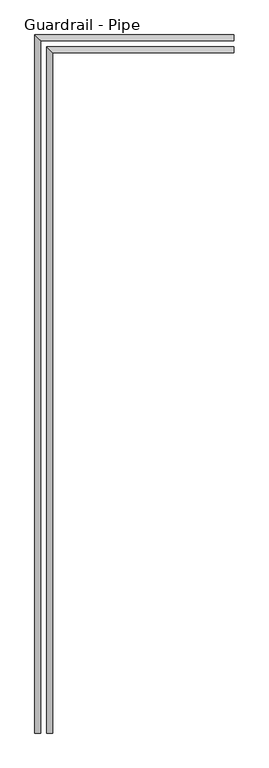
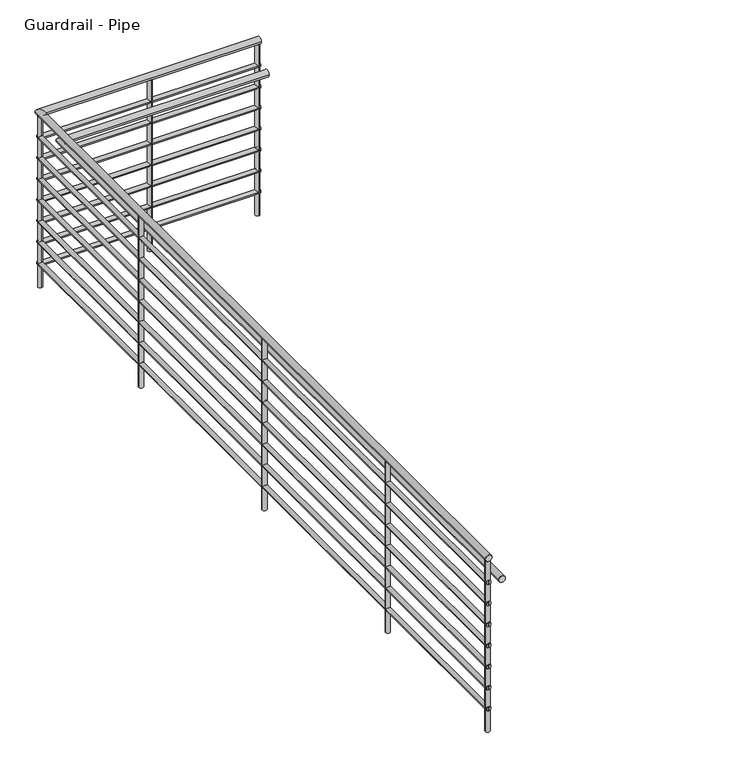
"""IFC4 building model written with IfcOpenShell, lengths in millimetres: railing geometry, Guardrail - Pipe."""

from ifc_helpers import new_model, si_unit, point, frame, frame_2d, origin, origin_with_axes, place, context, project, spatial, circle_curve, ellipse_curve, trimmed, segment, composite_curve, outline, extrude, source, transform, mapped, element, save
from ifc_brep_helpers import plane_surface, cylinder_surface, advanced_brep


def guardrail_pipe_2ce98fbd(model_context):
    return source(origin(), model_context, "Body", "SolidModel", [
        advanced_brep(
        [(-2073.0939612, 2865.859643, 1047.75), (-2073.0939612, 2903.959643, 1047.75), (-3304.9939612, 2865.859643, 1047.75), (-3343.0939612, 2903.959643, 1047.75), (-3304.9939612, -1546.6414366, 1047.75), (-3343.0939612, -1546.6414366, 1047.75)],
        [
            (0, 1, circle_curve(frame((-2073.0939612, 2884.909643, 1047.75), z_axis=(1.0, 0.0, 0.0), x_axis=(0.0, 1.0, 0.0)), 19.05)),
            (1, 0, circle_curve(frame((-2073.0939612, 2884.909643, 1047.75), z_axis=(1.0, 0.0, 0.0), x_axis=(0.0, 1.0, 0.0)), 19.05)),
            (0, 2),
            (2, 3, ellipse_curve(frame((-3324.0439612, 2884.909643, 1047.75), z_axis=(0.7071067811865492, 0.7071067811865458, 0.0), x_axis=(0.7071067811865458, -0.7071067811865492, 0.0)), 26.9407684, 19.05)),
            (3, 1),
            (3, 2, ellipse_curve(frame((-3324.0439612, 2884.909643, 1047.75), z_axis=(0.7071067811865492, 0.7071067811865458, 0.0), x_axis=(0.7071067811865458, -0.7071067811865492, 0.0)), 26.9407684, 19.05)),
            (4, 5, circle_curve(frame((-3324.0439612, -1546.6414366, 1047.75), z_axis=(0.0, -1.0, 0.0), x_axis=(-1.0, 0.0, 0.0)), 19.05)),
            (5, 4, circle_curve(frame((-3324.0439612, -1546.6414366, 1047.75), z_axis=(0.0, -1.0, 0.0), x_axis=(-1.0, 0.0, 0.0)), 19.05)),
            (2, 4),
            (5, 3),
        ],
        [
            plane_surface(frame((-2073.0939612, 2884.909643, 1066.8), z_axis=(1.0, 0.0, 0.0), x_axis=(0.0, -1.0, 0.0))),
            cylinder_surface(frame((-2073.0939612, 2884.909643, 1047.75), z_axis=(1.0, 0.0, 0.0), x_axis=(0.0, 1.0, 0.0)), 19.05),
            plane_surface(frame((-3324.0439612, -1546.6414366, 1066.8), z_axis=(0.0, -1.0, 0.0), x_axis=(0.0, 0.0, -1.0))),
            cylinder_surface(frame((-3324.0439612, 2884.909643, 1047.75), z_axis=(0.0, 1.0, 0.0), x_axis=(-1.0, 0.0, 0.0)), 19.05),
        ],
        [
            (0, [[1, 2]]),
            (1, [[-1, 3, 4, 5]]),
            (1, [[-2, -5, 6, -3]]),
            (2, [[7, 8]]),
            (3, [[-4, 9, -8, 10]]),
            (3, [[-6, -10, -7, -9]]),
        ],
    ),
        advanced_brep(
        [(-2073.0939612, 2872.209643, 901.7), (-2073.0939612, 2897.609643, 901.7), (-3311.3439612, 2872.209643, 901.7), (-3336.7439612, 2897.609643, 901.7), (-3311.3439612, -1546.6414366, 901.7), (-3336.7439612, -1546.6414366, 901.7)],
        [
            (0, 1, circle_curve(frame((-2073.0939612, 2884.909643, 901.7), z_axis=(1.0, 0.0, 0.0), x_axis=(0.0, 1.0, 0.0)), 12.7)),
            (1, 0, circle_curve(frame((-2073.0939612, 2884.909643, 901.7), z_axis=(1.0, 0.0, 0.0), x_axis=(0.0, 1.0, 0.0)), 12.7)),
            (0, 2),
            (2, 3, ellipse_curve(frame((-3324.0439612, 2884.909643, 901.7), z_axis=(0.7071067811865492, 0.7071067811865458, 0.0), x_axis=(0.7071067811865458, -0.7071067811865492, 0.0)), 17.9605122, 12.7)),
            (3, 1),
            (3, 2, ellipse_curve(frame((-3324.0439612, 2884.909643, 901.7), z_axis=(0.7071067811865492, 0.7071067811865458, 0.0), x_axis=(0.7071067811865458, -0.7071067811865492, 0.0)), 17.9605122, 12.7)),
            (4, 5, circle_curve(frame((-3324.0439612, -1546.6414366, 901.7), z_axis=(0.0, -1.0, 0.0), x_axis=(-1.0, 0.0, 0.0)), 12.7)),
            (5, 4, circle_curve(frame((-3324.0439612, -1546.6414366, 901.7), z_axis=(0.0, -1.0, 0.0), x_axis=(-1.0, 0.0, 0.0)), 12.7)),
            (2, 4),
            (5, 3),
        ],
        [
            plane_surface(frame((-2073.0939612, 2884.909643, 914.4), z_axis=(1.0, 0.0, 0.0), x_axis=(0.0, -1.0, 0.0))),
            cylinder_surface(frame((-2073.0939612, 2884.909643, 901.7), z_axis=(1.0, 0.0, 0.0), x_axis=(0.0, 1.0, 0.0)), 12.7),
            plane_surface(frame((-3324.0439612, -1546.6414366, 914.4), z_axis=(0.0, -1.0, 0.0), x_axis=(0.0, 0.0, -1.0))),
            cylinder_surface(frame((-3324.0439612, 2884.909643, 901.7), z_axis=(0.0, 1.0, 0.0), x_axis=(-1.0, 0.0, 0.0)), 12.7),
        ],
        [
            (0, [[1, 2]]),
            (1, [[-1, 3, 4, 5]]),
            (1, [[-2, -5, 6, -3]]),
            (2, [[7, 8]]),
            (3, [[-4, 9, -8, 10]]),
            (3, [[-6, -10, -7, -9]]),
        ],
    ),
        advanced_brep(
        [(-2073.0939612, 2789.659643, 895.35), (-2073.0939612, 2827.759643, 895.35), (-3228.7939612, 2789.659643, 895.35), (-3266.8939612, 2827.759643, 895.35), (-3228.7939612, -1546.6414366, 895.35), (-3266.8939612, -1546.6414366, 895.35)],
        [
            (0, 1, circle_curve(frame((-2073.0939612, 2808.709643, 895.35), z_axis=(1.0, 0.0, 0.0), x_axis=(0.0, 1.0, 0.0)), 19.05)),
            (1, 0, circle_curve(frame((-2073.0939612, 2808.709643, 895.35), z_axis=(1.0, 0.0, 0.0), x_axis=(0.0, 1.0, 0.0)), 19.05)),
            (0, 2),
            (2, 3, ellipse_curve(frame((-3247.8439612, 2808.709643, 895.35), z_axis=(0.7071067811865492, 0.7071067811865458, 0.0), x_axis=(0.7071067811865458, -0.7071067811865492, 0.0)), 26.9407684, 19.05)),
            (3, 1),
            (3, 2, ellipse_curve(frame((-3247.8439612, 2808.709643, 895.35), z_axis=(0.7071067811865492, 0.7071067811865458, 0.0), x_axis=(0.7071067811865458, -0.7071067811865492, 0.0)), 26.9407684, 19.05)),
            (4, 5, circle_curve(frame((-3247.8439612, -1546.6414366, 895.35), z_axis=(0.0, -1.0, 0.0), x_axis=(-1.0, 0.0, 0.0)), 19.05)),
            (5, 4, circle_curve(frame((-3247.8439612, -1546.6414366, 895.35), z_axis=(0.0, -1.0, 0.0), x_axis=(-1.0, 0.0, 0.0)), 19.05)),
            (2, 4),
            (5, 3),
        ],
        [
            plane_surface(frame((-2073.0939612, 2808.709643, 914.4), z_axis=(1.0, 0.0, 0.0), x_axis=(0.0, -1.0, 0.0))),
            cylinder_surface(frame((-2073.0939612, 2808.709643, 895.35), z_axis=(1.0, 0.0, 0.0), x_axis=(0.0, 1.0, 0.0)), 19.05),
            plane_surface(frame((-3247.8439612, -1546.6414366, 914.4), z_axis=(0.0, -1.0, 0.0), x_axis=(0.0, 0.0, -1.0))),
            cylinder_surface(frame((-3247.8439612, 2808.709643, 895.35), z_axis=(0.0, 1.0, 0.0), x_axis=(-1.0, 0.0, 0.0)), 19.05),
        ],
        [
            (0, [[1, 2]]),
            (1, [[-1, 3, 4, 5]]),
            (1, [[-2, -5, 6, -3]]),
            (2, [[7, 8]]),
            (3, [[-4, 9, -8, 10]]),
            (3, [[-6, -10, -7, -9]]),
        ],
    ),
        advanced_brep(
        [(-2073.0939612, 2872.209643, 774.7), (-2073.0939612, 2897.609643, 774.7), (-3311.3439612, 2872.209643, 774.7), (-3336.7439612, 2897.609643, 774.7), (-3311.3439612, -1546.6414366, 774.7), (-3336.7439612, -1546.6414366, 774.7)],
        [
            (0, 1, circle_curve(frame((-2073.0939612, 2884.909643, 774.7), z_axis=(1.0, 0.0, 0.0), x_axis=(0.0, 1.0, 0.0)), 12.7)),
            (1, 0, circle_curve(frame((-2073.0939612, 2884.909643, 774.7), z_axis=(1.0, 0.0, 0.0), x_axis=(0.0, 1.0, 0.0)), 12.7)),
            (0, 2),
            (2, 3, ellipse_curve(frame((-3324.0439612, 2884.909643, 774.7), z_axis=(0.7071067811865492, 0.7071067811865458, 0.0), x_axis=(0.7071067811865458, -0.7071067811865492, 0.0)), 17.9605122, 12.7)),
            (3, 1),
            (3, 2, ellipse_curve(frame((-3324.0439612, 2884.909643, 774.7), z_axis=(0.7071067811865492, 0.7071067811865458, 0.0), x_axis=(0.7071067811865458, -0.7071067811865492, 0.0)), 17.9605122, 12.7)),
            (4, 5, circle_curve(frame((-3324.0439612, -1546.6414366, 774.7), z_axis=(0.0, -1.0, 0.0), x_axis=(-1.0, 0.0, 0.0)), 12.7)),
            (5, 4, circle_curve(frame((-3324.0439612, -1546.6414366, 774.7), z_axis=(0.0, -1.0, 0.0), x_axis=(-1.0, 0.0, 0.0)), 12.7)),
            (2, 4),
            (5, 3),
        ],
        [
            plane_surface(frame((-2073.0939612, 2884.909643, 787.4), z_axis=(1.0, 0.0, 0.0), x_axis=(0.0, -1.0, 0.0))),
            cylinder_surface(frame((-2073.0939612, 2884.909643, 774.7), z_axis=(1.0, 0.0, 0.0), x_axis=(0.0, 1.0, 0.0)), 12.7),
            plane_surface(frame((-3324.0439612, -1546.6414366, 787.4), z_axis=(0.0, -1.0, 0.0), x_axis=(0.0, 0.0, -1.0))),
            cylinder_surface(frame((-3324.0439612, 2884.909643, 774.7), z_axis=(0.0, 1.0, 0.0), x_axis=(-1.0, 0.0, 0.0)), 12.7),
        ],
        [
            (0, [[1, 2]]),
            (1, [[-1, 3, 4, 5]]),
            (1, [[-2, -5, 6, -3]]),
            (2, [[7, 8]]),
            (3, [[-4, 9, -8, 10]]),
            (3, [[-6, -10, -7, -9]]),
        ],
    ),
        advanced_brep(
        [(-2073.0939612, 2872.209643, 647.7), (-2073.0939612, 2897.609643, 647.7), (-3311.3439612, 2872.209643, 647.7), (-3336.7439612, 2897.609643, 647.7), (-3311.3439612, -1546.6414366, 647.7), (-3336.7439612, -1546.6414366, 647.7)],
        [
            (0, 1, circle_curve(frame((-2073.0939612, 2884.909643, 647.7), z_axis=(1.0, 0.0, 0.0), x_axis=(0.0, 1.0, 0.0)), 12.7)),
            (1, 0, circle_curve(frame((-2073.0939612, 2884.909643, 647.7), z_axis=(1.0, 0.0, 0.0), x_axis=(0.0, 1.0, 0.0)), 12.7)),
            (0, 2),
            (2, 3, ellipse_curve(frame((-3324.0439612, 2884.909643, 647.7), z_axis=(0.7071067811865492, 0.7071067811865458, 0.0), x_axis=(0.7071067811865458, -0.7071067811865492, 0.0)), 17.9605122, 12.7)),
            (3, 1),
            (3, 2, ellipse_curve(frame((-3324.0439612, 2884.909643, 647.7), z_axis=(0.7071067811865492, 0.7071067811865458, 0.0), x_axis=(0.7071067811865458, -0.7071067811865492, 0.0)), 17.9605122, 12.7)),
            (4, 5, circle_curve(frame((-3324.0439612, -1546.6414366, 647.7), z_axis=(0.0, -1.0, 0.0), x_axis=(-1.0, 0.0, 0.0)), 12.7)),
            (5, 4, circle_curve(frame((-3324.0439612, -1546.6414366, 647.7), z_axis=(0.0, -1.0, 0.0), x_axis=(-1.0, 0.0, 0.0)), 12.7)),
            (2, 4),
            (5, 3),
        ],
        [
            plane_surface(frame((-2073.0939612, 2884.909643, 660.4), z_axis=(1.0, 0.0, 0.0), x_axis=(0.0, -1.0, 0.0))),
            cylinder_surface(frame((-2073.0939612, 2884.909643, 647.7), z_axis=(1.0, 0.0, 0.0), x_axis=(0.0, 1.0, 0.0)), 12.7),
            plane_surface(frame((-3324.0439612, -1546.6414366, 660.4), z_axis=(0.0, -1.0, 0.0), x_axis=(0.0, 0.0, -1.0))),
            cylinder_surface(frame((-3324.0439612, 2884.909643, 647.7), z_axis=(0.0, 1.0, 0.0), x_axis=(-1.0, 0.0, 0.0)), 12.7),
        ],
        [
            (0, [[1, 2]]),
            (1, [[-1, 3, 4, 5]]),
            (1, [[-2, -5, 6, -3]]),
            (2, [[7, 8]]),
            (3, [[-4, 9, -8, 10]]),
            (3, [[-6, -10, -7, -9]]),
        ],
    ),
        advanced_brep(
        [(-2073.0939612, 2872.209643, 520.7), (-2073.0939612, 2897.609643, 520.7), (-3311.3439612, 2872.209643, 520.7), (-3336.7439612, 2897.609643, 520.7), (-3311.3439612, -1546.6414366, 520.7), (-3336.7439612, -1546.6414366, 520.7)],
        [
            (0, 1, circle_curve(frame((-2073.0939612, 2884.909643, 520.7), z_axis=(1.0, 0.0, 0.0), x_axis=(0.0, 1.0, 0.0)), 12.7)),
            (1, 0, circle_curve(frame((-2073.0939612, 2884.909643, 520.7), z_axis=(1.0, 0.0, 0.0), x_axis=(0.0, 1.0, 0.0)), 12.7)),
            (0, 2),
            (2, 3, ellipse_curve(frame((-3324.0439612, 2884.909643, 520.7), z_axis=(0.7071067811865492, 0.7071067811865458, 0.0), x_axis=(0.7071067811865458, -0.7071067811865492, 0.0)), 17.9605122, 12.7)),
            (3, 1),
            (3, 2, ellipse_curve(frame((-3324.0439612, 2884.909643, 520.7), z_axis=(0.7071067811865492, 0.7071067811865458, 0.0), x_axis=(0.7071067811865458, -0.7071067811865492, 0.0)), 17.9605122, 12.7)),
            (4, 5, circle_curve(frame((-3324.0439612, -1546.6414366, 520.7), z_axis=(0.0, -1.0, 0.0), x_axis=(-1.0, 0.0, 0.0)), 12.7)),
            (5, 4, circle_curve(frame((-3324.0439612, -1546.6414366, 520.7), z_axis=(0.0, -1.0, 0.0), x_axis=(-1.0, 0.0, 0.0)), 12.7)),
            (2, 4),
            (5, 3),
        ],
        [
            plane_surface(frame((-2073.0939612, 2884.909643, 533.4), z_axis=(1.0, 0.0, 0.0), x_axis=(0.0, -1.0, 0.0))),
            cylinder_surface(frame((-2073.0939612, 2884.909643, 520.7), z_axis=(1.0, 0.0, 0.0), x_axis=(0.0, 1.0, 0.0)), 12.7),
            plane_surface(frame((-3324.0439612, -1546.6414366, 533.4), z_axis=(0.0, -1.0, 0.0), x_axis=(0.0, 0.0, -1.0))),
            cylinder_surface(frame((-3324.0439612, 2884.909643, 520.7), z_axis=(0.0, 1.0, 0.0), x_axis=(-1.0, 0.0, 0.0)), 12.7),
        ],
        [
            (0, [[1, 2]]),
            (1, [[-1, 3, 4, 5]]),
            (1, [[-2, -5, 6, -3]]),
            (2, [[7, 8]]),
            (3, [[-4, 9, -8, 10]]),
            (3, [[-6, -10, -7, -9]]),
        ],
    ),
        advanced_brep(
        [(-2073.0939612, 2872.209643, 393.7), (-2073.0939612, 2897.609643, 393.7), (-3311.3439612, 2872.209643, 393.7), (-3336.7439612, 2897.609643, 393.7), (-3311.3439612, -1546.6414366, 393.7), (-3336.7439612, -1546.6414366, 393.7)],
        [
            (0, 1, circle_curve(frame((-2073.0939612, 2884.909643, 393.7), z_axis=(1.0, 0.0, 0.0), x_axis=(0.0, 1.0, 0.0)), 12.7)),
            (1, 0, circle_curve(frame((-2073.0939612, 2884.909643, 393.7), z_axis=(1.0, 0.0, 0.0), x_axis=(0.0, 1.0, 0.0)), 12.7)),
            (0, 2),
            (2, 3, ellipse_curve(frame((-3324.0439612, 2884.909643, 393.7), z_axis=(0.7071067811865492, 0.7071067811865458, 0.0), x_axis=(0.7071067811865458, -0.7071067811865492, 0.0)), 17.9605122, 12.7)),
            (3, 1),
            (3, 2, ellipse_curve(frame((-3324.0439612, 2884.909643, 393.7), z_axis=(0.7071067811865492, 0.7071067811865458, 0.0), x_axis=(0.7071067811865458, -0.7071067811865492, 0.0)), 17.9605122, 12.7)),
            (4, 5, circle_curve(frame((-3324.0439612, -1546.6414366, 393.7), z_axis=(0.0, -1.0, 0.0), x_axis=(-1.0, 0.0, 0.0)), 12.7)),
            (5, 4, circle_curve(frame((-3324.0439612, -1546.6414366, 393.7), z_axis=(0.0, -1.0, 0.0), x_axis=(-1.0, 0.0, 0.0)), 12.7)),
            (2, 4),
            (5, 3),
        ],
        [
            plane_surface(frame((-2073.0939612, 2884.909643, 406.4), z_axis=(1.0, 0.0, 0.0), x_axis=(0.0, -1.0, 0.0))),
            cylinder_surface(frame((-2073.0939612, 2884.909643, 393.7), z_axis=(1.0, 0.0, 0.0), x_axis=(0.0, 1.0, 0.0)), 12.7),
            plane_surface(frame((-3324.0439612, -1546.6414366, 406.4), z_axis=(0.0, -1.0, 0.0), x_axis=(0.0, 0.0, -1.0))),
            cylinder_surface(frame((-3324.0439612, 2884.909643, 393.7), z_axis=(0.0, 1.0, 0.0), x_axis=(-1.0, 0.0, 0.0)), 12.7),
        ],
        [
            (0, [[1, 2]]),
            (1, [[-1, 3, 4, 5]]),
            (1, [[-2, -5, 6, -3]]),
            (2, [[7, 8]]),
            (3, [[-4, 9, -8, 10]]),
            (3, [[-6, -10, -7, -9]]),
        ],
    ),
        advanced_brep(
        [(-2073.0939612, 2872.209643, 266.7), (-2073.0939612, 2897.609643, 266.7), (-3311.3439612, 2872.209643, 266.7), (-3336.7439612, 2897.609643, 266.7), (-3311.3439612, -1546.6414366, 266.7), (-3336.7439612, -1546.6414366, 266.7)],
        [
            (0, 1, circle_curve(frame((-2073.0939612, 2884.909643, 266.7), z_axis=(1.0, 0.0, 0.0), x_axis=(0.0, 1.0, 0.0)), 12.7)),
            (1, 0, circle_curve(frame((-2073.0939612, 2884.909643, 266.7), z_axis=(1.0, 0.0, 0.0), x_axis=(0.0, 1.0, 0.0)), 12.7)),
            (0, 2),
            (2, 3, ellipse_curve(frame((-3324.0439612, 2884.909643, 266.7), z_axis=(0.7071067811865492, 0.7071067811865458, 0.0), x_axis=(0.7071067811865458, -0.7071067811865492, 0.0)), 17.9605122, 12.7)),
            (3, 1),
            (3, 2, ellipse_curve(frame((-3324.0439612, 2884.909643, 266.7), z_axis=(0.7071067811865492, 0.7071067811865458, 0.0), x_axis=(0.7071067811865458, -0.7071067811865492, 0.0)), 17.9605122, 12.7)),
            (4, 5, circle_curve(frame((-3324.0439612, -1546.6414366, 266.7), z_axis=(0.0, -1.0, 0.0), x_axis=(-1.0, 0.0, 0.0)), 12.7)),
            (5, 4, circle_curve(frame((-3324.0439612, -1546.6414366, 266.7), z_axis=(0.0, -1.0, 0.0), x_axis=(-1.0, 0.0, 0.0)), 12.7)),
            (2, 4),
            (5, 3),
        ],
        [
            plane_surface(frame((-2073.0939612, 2884.909643, 279.4), z_axis=(1.0, 0.0, 0.0), x_axis=(0.0, -1.0, 0.0))),
            cylinder_surface(frame((-2073.0939612, 2884.909643, 266.7), z_axis=(1.0, 0.0, 0.0), x_axis=(0.0, 1.0, 0.0)), 12.7),
            plane_surface(frame((-3324.0439612, -1546.6414366, 279.4), z_axis=(0.0, -1.0, 0.0), x_axis=(0.0, 0.0, -1.0))),
            cylinder_surface(frame((-3324.0439612, 2884.909643, 266.7), z_axis=(0.0, 1.0, 0.0), x_axis=(-1.0, 0.0, 0.0)), 12.7),
        ],
        [
            (0, [[1, 2]]),
            (1, [[-1, 3, 4, 5]]),
            (1, [[-2, -5, 6, -3]]),
            (2, [[7, 8]]),
            (3, [[-4, 9, -8, 10]]),
            (3, [[-6, -10, -7, -9]]),
        ],
    ),
        advanced_brep(
        [(-2073.0939612, 2872.209643, 139.7), (-2073.0939612, 2897.609643, 139.7), (-3311.3439612, 2872.209643, 139.7), (-3336.7439612, 2897.609643, 139.7), (-3311.3439612, -1546.6414366, 139.7), (-3336.7439612, -1546.6414366, 139.7)],
        [
            (0, 1, circle_curve(frame((-2073.0939612, 2884.909643, 139.7), z_axis=(1.0, 0.0, 0.0), x_axis=(0.0, 1.0, 0.0)), 12.7)),
            (1, 0, circle_curve(frame((-2073.0939612, 2884.909643, 139.7), z_axis=(1.0, 0.0, 0.0), x_axis=(0.0, 1.0, 0.0)), 12.7)),
            (0, 2),
            (2, 3, ellipse_curve(frame((-3324.0439612, 2884.909643, 139.7), z_axis=(0.7071067811865492, 0.7071067811865458, 0.0), x_axis=(0.7071067811865458, -0.7071067811865492, 0.0)), 17.9605122, 12.7)),
            (3, 1),
            (3, 2, ellipse_curve(frame((-3324.0439612, 2884.909643, 139.7), z_axis=(0.7071067811865492, 0.7071067811865458, 0.0), x_axis=(0.7071067811865458, -0.7071067811865492, 0.0)), 17.9605122, 12.7)),
            (4, 5, circle_curve(frame((-3324.0439612, -1546.6414366, 139.7), z_axis=(0.0, -1.0, 0.0), x_axis=(-1.0, 0.0, 0.0)), 12.7)),
            (5, 4, circle_curve(frame((-3324.0439612, -1546.6414366, 139.7), z_axis=(0.0, -1.0, 0.0), x_axis=(-1.0, 0.0, 0.0)), 12.7)),
            (2, 4),
            (5, 3),
        ],
        [
            plane_surface(frame((-2073.0939612, 2884.909643, 152.4), z_axis=(1.0, 0.0, 0.0), x_axis=(0.0, -1.0, 0.0))),
            cylinder_surface(frame((-2073.0939612, 2884.909643, 139.7), z_axis=(1.0, 0.0, 0.0), x_axis=(0.0, 1.0, 0.0)), 12.7),
            plane_surface(frame((-3324.0439612, -1546.6414366, 152.4), z_axis=(0.0, -1.0, 0.0), x_axis=(0.0, 0.0, -1.0))),
            cylinder_surface(frame((-3324.0439612, 2884.909643, 139.7), z_axis=(0.0, 1.0, 0.0), x_axis=(-1.0, 0.0, 0.0)), 12.7),
        ],
        [
            (0, [[1, 2]]),
            (1, [[-1, 3, 4, 5]]),
            (1, [[-2, -5, 6, -3]]),
            (2, [[7, 8]]),
            (3, [[-4, 9, -8, 10]]),
            (3, [[-6, -10, -7, -9]]),
        ],
    ),
        extrude(outline(composite_curve([segment(trimmed(circle_curve(frame_2d((-3324.0439612, -550.0658968)), 12.7), [point((-3336.7439612, -550.0658968))], [point((-3311.3439612, -550.0658968))], False, "CARTESIAN"), True, "CONTINUOUS"), segment(trimmed(circle_curve(frame_2d((-3324.0439612, -550.0658968)), 12.7), [point((-3311.3439612, -550.0658968))], [point((-3336.7439612, -550.0658968))], False, "CARTESIAN"), True, "CONTINUOUS")], self_intersect=False)), origin_with_axes(), (0.0, 0.0, 1.0), 1028.7),
        extrude(outline(composite_curve([segment(trimmed(circle_curve(frame_2d((-3324.0439612, 669.1341032)), 12.7), [point((-3336.7439612, 669.1341032))], [point((-3311.3439612, 669.1341032))], False, "CARTESIAN"), True, "CONTINUOUS"), segment(trimmed(circle_curve(frame_2d((-3324.0439612, 669.1341032)), 12.7), [point((-3311.3439612, 669.1341032))], [point((-3336.7439612, 669.1341032))], False, "CARTESIAN"), True, "CONTINUOUS")], self_intersect=False)), origin_with_axes(), (0.0, 0.0, 1.0), 1028.7),
        extrude(outline(composite_curve([segment(trimmed(circle_curve(frame_2d((-3324.0439612, 1888.3341032)), 12.7), [point((-3336.7439612, 1888.3341032))], [point((-3311.3439612, 1888.3341032))], False, "CARTESIAN"), True, "CONTINUOUS"), segment(trimmed(circle_curve(frame_2d((-3324.0439612, 1888.3341032)), 12.7), [point((-3311.3439612, 1888.3341032))], [point((-3336.7439612, 1888.3341032))], False, "CARTESIAN"), True, "CONTINUOUS")], self_intersect=False)), origin_with_axes(), (0.0, 0.0, 1.0), 1028.7),
        extrude(outline(composite_curve([segment(trimmed(circle_curve(frame_2d((-2698.5689612, 2884.909643)), 12.7), [point((-2698.5689612, 2897.609643))], [point((-2698.5689612, 2872.209643))], False, "CARTESIAN"), True, "CONTINUOUS"), segment(trimmed(circle_curve(frame_2d((-2698.5689612, 2884.909643)), 12.7), [point((-2698.5689612, 2872.209643))], [point((-2698.5689612, 2897.609643))], False, "CARTESIAN"), True, "CONTINUOUS")], self_intersect=False)), origin_with_axes(), (0.0, 0.0, 1.0), 1028.7),
        extrude(outline(composite_curve([segment(trimmed(circle_curve(frame_2d((-3324.0439612, 2884.909643)), 12.7), [point((-3324.0439612, 2897.609643))], [point((-3324.0439612, 2872.209643))], False, "CARTESIAN"), True, "CONTINUOUS"), segment(trimmed(circle_curve(frame_2d((-3324.0439612, 2884.909643)), 12.7), [point((-3324.0439612, 2872.209643))], [point((-3324.0439612, 2897.609643))], False, "CARTESIAN"), True, "CONTINUOUS")], self_intersect=False)), origin_with_axes(), (0.0, 0.0, 1.0), 1028.7),
        extrude(outline(composite_curve([segment(trimmed(circle_curve(frame_2d((-3324.0439612, -1534.2598521)), 12.7), [point((-3336.7439612, -1534.2598521))], [point((-3311.3439612, -1534.2598521))], False, "CARTESIAN"), True, "CONTINUOUS"), segment(trimmed(circle_curve(frame_2d((-3324.0439612, -1534.2598521)), 12.7), [point((-3311.3439612, -1534.2598521))], [point((-3336.7439612, -1534.2598521))], False, "CARTESIAN"), True, "CONTINUOUS")], self_intersect=False)), origin_with_axes(), (0.0, 0.0, 1.0), 1028.7),
        extrude(outline(composite_curve([segment(trimmed(circle_curve(frame_2d((-2085.4755457, 2884.909643)), 12.7), [point((-2085.4755457, 2897.609643))], [point((-2085.4755457, 2872.209643))], False, "CARTESIAN"), True, "CONTINUOUS"), segment(trimmed(circle_curve(frame_2d((-2085.4755457, 2884.909643)), 12.7), [point((-2085.4755457, 2872.209643))], [point((-2085.4755457, 2897.609643))], False, "CARTESIAN"), True, "CONTINUOUS")], self_intersect=False)), origin_with_axes(), (0.0, 0.0, 1.0), 1028.7),
    ])


if __name__ == "__main__":
    model = new_model("IFC4")
    model_context = context("Model", 3, world=origin())
    ifc_project = project(units=[si_unit("LENGTHUNIT", "METRE", prefix="MILLI")], contexts=[model_context])
    site = spatial("IfcSite", under=ifc_project)
    building = spatial("IfcBuilding", under=site)
    placement = place(None, origin())
    guardrail_pipe_shape = guardrail_pipe_2ce98fbd(model_context)
    element("IfcRailing", 1, ObjectType="Guardrail - Pipe", at=placement, inside=building, context=model_context, shape_type="MappedRepresentation", body=[
        mapped(guardrail_pipe_shape, transform((0.0, 0.0, 0.0), x_axis=(1.0, 0.0, 0.0), y_axis=(0.0, 1.0, 0.0), z_axis=(0.0, 0.0, 1.0))),
    ])
    save(model, "model.ifc")

# Revit data of these elements
# Element 1 (IfcRailing, "Guardrail - Pipe")
#   Materials on its faces: "Metal - Aluminum", "Metal - Steel"
# Materials
#   "Metal - Aluminum": class "Metal", colour RGB 244 244 244, transparency 0, Comments = "Rendering appearance not upgraded Rendering appearance not upgraded ", Description = "Aluminum"
#   "Metal - Steel": class "Metal", colour RGB 76 76 76, transparency 0, Comments = "Rendering appearance not upgraded Rendering appearance not upgraded ", Description = "Steel"
